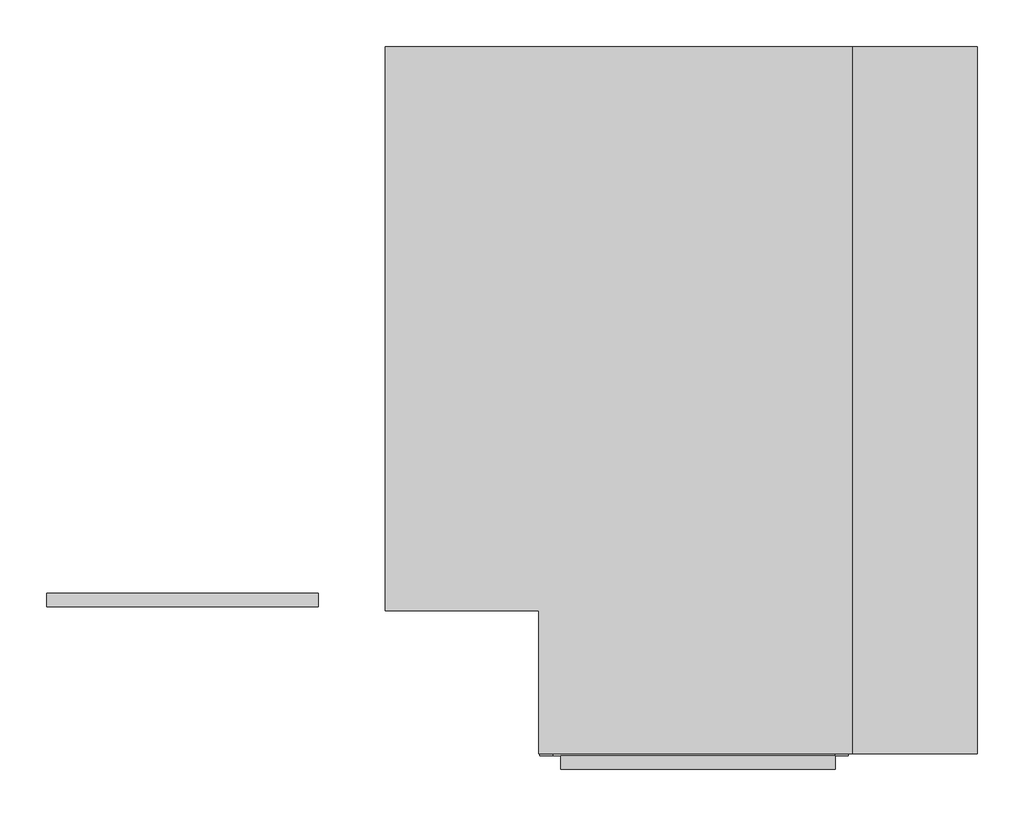
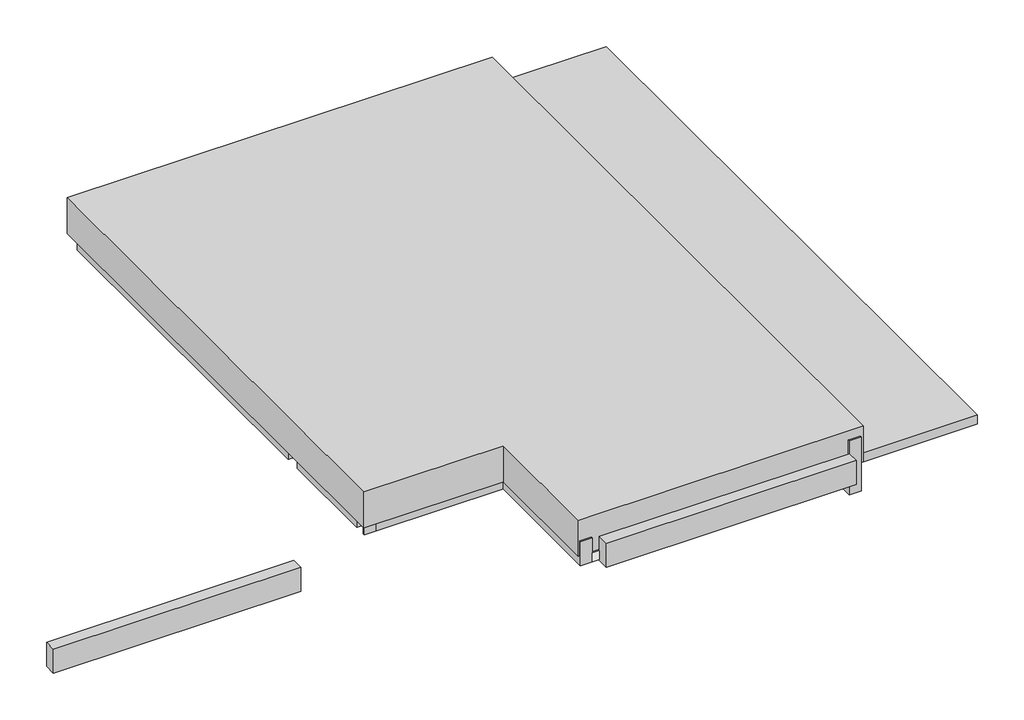
# One storey: 7 beams, 2 proxies, 2 slabs, 1 column.
"""IFC4 building model written with IfcOpenShell, lengths in millimetres."""

import ifcopenshell
import ifcopenshell.guid

model = None  # the IFC model being written
_history = None  # IfcOwnerHistory: only IFC2X3 demands one
_inside = {}  # id of a spatial element -> (the spatial element, [elements in it])
_under = {}  # id of a project, library or spatial element -> (it, [spatial elements below it])
_declared = {}  # id of a project -> (the project, [libraries it declares])
_typed = {}  # id of a type object -> (the type object, [elements of that type])
_made_of = {}  # id of a material, layer set ... -> (it, [elements and type objects made of it])


def new_model(schema):
    """Start an empty IFC model of exactly this schema.

    Asked for "IFC4X3", IfcOpenShell would pick the latest addendum, in which some entities
    have other attributes; the version numbers below select the first issue.
    IFC2X3 requires an IfcOwnerHistory on every rooted entity: one is made here for all.
    """
    global model, _history
    if schema == "IFC4X3":
        model = ifcopenshell.file(schema_version=(4, 3, 0, 0))
    else:
        model = ifcopenshell.file(schema=schema)
    _inside.clear()
    _under.clear()
    _declared.clear()
    _typed.clear()
    _made_of.clear()
    _history = None
    if model.schema == "IFC2X3":
        org = make("IfcOrganization", Name="unknown")
        user = make(
            "IfcPersonAndOrganization",
            ThePerson=make("IfcPerson", FamilyName="unknown"),
            TheOrganization=org,
        )
        app = make(
            "IfcApplication",
            ApplicationDeveloper=org,
            Version="unknown",
            ApplicationFullName="unknown",
            ApplicationIdentifier="unknown",
        )
        _history = make(
            "IfcOwnerHistory",
            OwningUser=user,
            OwningApplication=app,
            ChangeAction="ADDED",
            CreationDate=0,
        )
    return model


def make(cls, **values):
    """One entity of the class cls with the attributes given. An attribute that is None is left unset."""
    return model.create_entity(
        cls, **{name: value for name, value in values.items() if value is not None}
    )


def rooted(cls, **values):
    """An entity with a GlobalId (a new one), such as an element, a storey or a relation."""
    return make(cls, GlobalId=ifcopenshell.guid.new(), OwnerHistory=_history, **values)


def si_unit(unit_type, name, prefix=None):
    """IfcSIUnit, for example si_unit("LENGTHUNIT", "METRE", prefix="MILLI")."""
    return make("IfcSIUnit", UnitType=unit_type, Prefix=prefix, Name=name)


def assignment(units):
    """IfcUnitAssignment: the units of a project."""
    return None if units is None else make("IfcUnitAssignment", Units=units)


def point(xyz):
    """IfcCartesianPoint."""
    return None if xyz is None else make("IfcCartesianPoint", Coordinates=xyz)


def direction(xyz):
    """IfcDirection."""
    return None if xyz is None else make("IfcDirection", DirectionRatios=xyz)


def frame(location, z_axis=None, x_axis=None):
    """IfcAxis2Placement3D, a coordinate frame: its origin and axes. An axis left out is left unset."""
    return make(
        "IfcAxis2Placement3D",
        Location=point(location),
        Axis=direction(z_axis),
        RefDirection=direction(x_axis),
    )


def origin():
    """The frame at (0, 0, 0) with its axes left unset."""
    return frame((0.0, 0.0, 0.0))


def place(relative_to, where):
    """IfcLocalPlacement: puts the frame where relative to a parent placement (None: the world)."""
    return make(
        "IfcLocalPlacement", PlacementRelTo=relative_to, RelativePlacement=where
    )


def context(
    kind, dimensions, precision=None, world=None, true_north=None, identifier=None
):
    """IfcGeometricRepresentationContext, for example the 3D "Model" context."""
    return make(
        "IfcGeometricRepresentationContext",
        ContextIdentifier=identifier,
        ContextType=kind,
        CoordinateSpaceDimension=dimensions,
        Precision=precision,
        WorldCoordinateSystem=world,
        TrueNorth=true_north,
    )


def project(units=None, contexts=None):
    """IfcProject with its units and contexts."""
    return rooted(
        "IfcProject",
        Name="project",
        RepresentationContexts=contexts,
        UnitsInContext=assignment(units),
    )


def spatial(cls, under=None, at=None, **own):
    """A site, building, storey or space (cls), placed at a placement, below another one or the project."""
    s = rooted(cls, ObjectPlacement=at, **own)
    if under is not None:
        _under.setdefault(under.id(), (under, []))[1].append(s)
    return s


def polyline(points):
    """IfcPolyline through the points."""
    return make("IfcPolyline", Points=[point(p) for p in points])


def outline(outer, holes=None, kind="AREA"):
    """IfcArbitraryClosedProfileDef: a profile drawn as a closed curve; with holes, ...WithVoids."""
    if holes is None:
        return make("IfcArbitraryClosedProfileDef", ProfileType=kind, OuterCurve=outer)
    return make(
        "IfcArbitraryProfileDefWithVoids",
        ProfileType=kind,
        OuterCurve=outer,
        InnerCurves=holes,
    )


def extrude(swept, where, along, depth):
    """IfcExtrudedAreaSolid: the profile swept, set in the frame where, extruded along a direction by depth."""
    return make(
        "IfcExtrudedAreaSolid",
        SweptArea=swept,
        Position=where,
        ExtrudedDirection=direction(along),
        Depth=depth,
    )


def faces_of(points, faces, orient=None, outer=None):
    """IfcFace entities. A face is a list of loops; a loop is a list of indices into points, from 0.

    orient and outer hold one flag for each loop. By default every Orientation is true, the
    first loop of a face is its IfcFaceOuterBound and the others are IfcFaceBound.
    """
    made = []
    for i, loops in enumerate(faces):
        bounds = []
        for j, loop in enumerate(loops):
            is_outer = j == 0 if outer is None else outer[i][j]
            bounds.append(
                make(
                    "IfcFaceOuterBound" if is_outer else "IfcFaceBound",
                    Bound=make("IfcPolyLoop", Polygon=[points[k] for k in loop]),
                    Orientation=True if orient is None else orient[i][j],
                )
            )
        made.append(make("IfcFace", Bounds=bounds))
    return made


def faceted_brep(points, faces, orient=None, outer=None, voids=None):
    """IfcFacetedBrep: a solid bounded by flat faces; with voids (closed shells), ...WithVoids."""
    shared = [point(p) for p in points]
    hull = make("IfcClosedShell", CfsFaces=faces_of(shared, faces, orient, outer))
    if voids is None:
        return make("IfcFacetedBrep", Outer=hull)
    return make(
        "IfcFacetedBrepWithVoids",
        Outer=hull,
        Voids=[
            make(cls, CfsFaces=faces_of(shared, fs, o, b)) for cls, fs, o, b in voids
        ],
    )


def shape(context_of_items, identifier, shape_type, items):
    """IfcShapeRepresentation: the items that make up one representation, for example the "Body"."""
    return make(
        "IfcShapeRepresentation",
        ContextOfItems=context_of_items,
        RepresentationIdentifier=identifier,
        RepresentationType=shape_type,
        Items=items,
    )


def source(mapping_origin, context_of_items, identifier, shape_type, items):
    """IfcRepresentationMap: a shape defined once, which mapped items show again and again."""
    return make(
        "IfcRepresentationMap",
        MappingOrigin=mapping_origin,
        MappedRepresentation=shape(context_of_items, identifier, shape_type, items),
    )


def transform(
    local_origin,
    x_axis=None,
    y_axis=None,
    z_axis=None,
    scale=None,
    scale2=None,
    scale3=None,
    uniform=True,
):
    """IfcCartesianTransformationOperator3D, or its non-uniform kind. x_axis, y_axis, z_axis: its Axis1, 2, 3."""
    if uniform:
        return make(
            "IfcCartesianTransformationOperator3D",
            Axis1=direction(x_axis),
            Axis2=direction(y_axis),
            LocalOrigin=point(local_origin),
            Scale=scale,
            Axis3=direction(z_axis),
        )
    return make(
        "IfcCartesianTransformationOperator3DnonUniform",
        Axis1=direction(x_axis),
        Axis2=direction(y_axis),
        LocalOrigin=point(local_origin),
        Scale=scale,
        Axis3=direction(z_axis),
        Scale2=scale2,
        Scale3=scale3,
    )


def mapped(mapping_source, mapping_target):
    """IfcMappedItem: shows the shape of a source again, moved by a transform."""
    return make(
        "IfcMappedItem", MappingSource=mapping_source, MappingTarget=mapping_target
    )


def made_of(thing, what):
    """Note that an element or type object is made of a material, layer set ...; save() writes the relation."""
    if what is not None:
        _made_of.setdefault(what.id(), (what, []))[1].append(thing)
    return thing


def element(
    cls,
    number,
    at=None,
    inside=None,
    cuts=None,
    type_object=None,
    material=None,
    context=None,
    identifier="Body",
    shape_type=None,
    held_by="IfcProductDefinitionShape",
    body=None,
    shapes=None,
    **own,
):
    """One element of the class cls, such as IfcWall. Its Tag is "e" and its number.

    at: its placement. inside: the storey or other place that contains it. cuts: it is an
    opening in that element (IfcRelVoidsElement). A single representation is given by context,
    identifier, shape_type and body (its items); several are given by shapes. held_by: the class
    of the entity that holds the representations. save() writes the other relations.
    """
    e = rooted(cls, Tag="e%d" % number, ObjectPlacement=at, **own)
    if body is not None:
        shapes = [shape(context, identifier, shape_type, body)]
    if shapes is not None:
        e.Representation = make(held_by, Representations=shapes)
    if inside is not None:
        _inside.setdefault(inside.id(), (inside, []))[1].append(e)
    if cuts is not None:
        rooted(
            "IfcRelVoidsElement", RelatingBuildingElement=cuts, RelatedOpeningElement=e
        )
    if type_object is not None:
        _typed.setdefault(type_object.id(), (type_object, []))[1].append(e)
    return made_of(e, material)


def aggregate(whole, parts):
    """IfcRelAggregates: a whole, such as a stair, and the parts it consists of."""
    return rooted("IfcRelAggregates", RelatingObject=whole, RelatedObjects=parts)


def save(model, path):
    """Write the relations noted so far, then the file.

    IfcRelAggregates (storeys below a building ...), IfcRelContainedInSpatialStructure (elements
    in a storey), IfcRelDefinesByType, IfcRelAssociatesMaterial and IfcRelDeclares: one each for
    every whole, place, type object, material and project.
    """
    for whole, parts in _under.values():
        aggregate(whole, parts)
    for where, things in _inside.values():
        rooted(
            "IfcRelContainedInSpatialStructure",
            RelatedElements=things,
            RelatingStructure=where,
        )
    for kind, things in _typed.values():
        rooted("IfcRelDefinesByType", RelatedObjects=things, RelatingType=kind)
    for what, things in _made_of.values():
        rooted("IfcRelAssociatesMaterial", RelatedObjects=things, RelatingMaterial=what)
    for by, libraries in _declared.values():
        rooted("IfcRelDeclares", RelatingContext=by, RelatedDefinitions=libraries)
    model.write(path)


def column_f3930958(model_context):
    return source(origin(), model_context, "Body", "SweptSolid", [
        extrude(outline(polyline([(30.0, 80.0), (30.0, -80.0), (-30.0, -80.0), (-30.0, 80.0), (30.0, 80.0)])), frame((0.0, 0.0, 4460.0), z_axis=(0.0, 0.0, 1.0), x_axis=(1.0, 0.0, 0.0)), (0.0, 0.0, 1.0), 522.9),
    ])


model = new_model("IFC4")

# Units and contexts
model_context = context("Model", 3, world=origin())
ifc_project = project(units=[si_unit("LENGTHUNIT", "METRE", prefix="MILLI")], contexts=[model_context])

# Site, building, storey
site = spatial("IfcSite", under=ifc_project)
building = spatial("IfcBuilding", under=site)
storey = spatial("IfcBuildingStorey", under=building, Name="COBERTURA SALA DE ESTAR", Elevation=4400.0)

# Beams
placement = place(None, origin())
element("IfcBeam", 1, ObjectType="TQS - Viga retangular : 19.0 x 40.0", at=placement, inside=storey, context=model_context, shape_type="SweptSolid", body=[
    extrude(outline(polyline([(-7621.281307, -2044.5699847), (-7621.281307, -2234.5699847), (-11521.281307, -2234.5699847), (-11521.281307, -2044.5699847), (-7621.281307, -2044.5699847)])), frame((0.0, 0.0, 3640.0), z_axis=(0.0, 0.0, 1.0), x_axis=(1.0, 0.0, 0.0)), (0.0, 0.0, 1.0), 400.0),
])
element("IfcBeam", 2, ObjectType="TQS - Viga retangular : 19.0 x 40.0", at=placement, inside=storey, context=model_context, shape_type="SweptSolid", body=[
    extrude(outline(polyline([(-202.281307, -4375.5699847), (-202.281307, -4565.5699847), (-4142.481307, -4565.5699847), (-4142.481307, -4375.5699847), (-202.281307, -4375.5699847)])), frame((0.0, 0.0, 4240.0), z_axis=(0.0, 0.0, 1.0), x_axis=(1.0, 0.0, 0.0)), (0.0, 0.0, 1.0), 400.0),
])
element("IfcBeam", 3, ObjectType="TQS - Viga retangular : 19.0 x 40.0", at=placement, inside=storey, context=model_context, shape_type="Brep", body=[
    faceted_brep([(-4442.481307, -2259.5699847, 4650.0), (-4252.481307, -2259.5699847, 4650.0), (-4252.481307, -2259.5699847, 4400.0), (-4252.481307, -2259.5699847, 4250.0), (-4442.481307, -2259.5699847, 4250.0), (-4442.481307, -4375.5699847, 4650.0), (-4252.481307, -4375.5699847, 4650.0), (-4252.481307, -4375.5699847, 4400.0), (-4252.481307, -4375.5699847, 4250.0), (-4442.481307, -4375.5699847, 4250.0)], [[[0, 1, 2, 3, 4]], [[1, 0, 5, 6]], [[3, 2, 1, 6, 7, 8]], [[4, 3, 8, 9]], [[0, 4, 9, 5]], [[5, 9, 8, 7, 6]]]),
])
element("IfcBeam", 4, ObjectType="TQS - Viga retangular : 19.0 x 60.0", at=placement, inside=storey, context=model_context, shape_type="SweptSolid", body=[
    extrude(outline(polyline([(-412.281307, 5584.4300153), (-6230.281307, 5584.4300153), (-6230.281307, 5774.4300153), (-412.281307, 5774.4300153), (-412.281307, 5584.4300153)])), frame((0.0, 0.0, 4250.0), z_axis=(0.0, 0.0, 1.0), x_axis=(1.0, 0.0, 0.0)), (0.0, 0.0, 1.0), 600.0),
])
element("IfcBeam", 5, ObjectType="TQS - Viga retangular : 19.0 x 60.0", at=placement, inside=storey, context=model_context, shape_type="Brep", body=[
    faceted_brep([(-6630.281307, -174.5699847, 4850.0), (-6440.281307, -174.5699847, 4850.0), (-6440.281307, 5584.4300153, 4850.0), (-6630.281307, 5584.4300153, 4850.0), (-6440.281307, -174.5699847, 4250.0), (-6440.281307, 5584.4300153, 4250.0), (-6440.281307, 5584.4300153, 4400.0), (-6630.281307, -174.5699847, 4250.0), (-6630.281307, 5584.4300153, 4250.0)], [[[0, 1, 2, 3]], [[1, 4, 5, 6, 2]], [[4, 7, 8, 5]], [[7, 0, 3, 8]], [[1, 0, 7, 4]], [[3, 2, 6, 5, 8]]]),
    faceted_brep([(-6630.281307, -424.5699847, 4850.0), (-6440.281307, -424.5699847, 4850.0), (-6440.281307, -424.5699847, 4250.0), (-6630.281307, -424.5699847, 4250.0), (-6630.281307, -2044.5699847, 4850.0), (-6440.281307, -2044.5699847, 4850.0), (-6440.281307, -2044.5699847, 4250.0), (-6630.281307, -2044.5699847, 4250.0)], [[[0, 1, 2, 3]], [[1, 0, 4, 5]], [[2, 1, 5, 6]], [[3, 2, 6, 7]], [[0, 3, 7, 4]], [[5, 4, 7, 6]]]),
    faceted_brep([(-6440.281307, -2259.5699847, 4850.0), (-6630.281307, -2259.5699847, 4850.0), (-6630.281307, -2259.5699847, 4250.0), (-6440.281307, -2259.5699847, 4250.0), (-6630.281307, -2234.5699847, 4850.0), (-6440.281307, -2234.5699847, 4850.0), (-6440.281307, -2234.5699847, 4250.0), (-6630.281307, -2234.5699847, 4250.0)], [[[0, 1, 2, 3]], [[4, 5, 6, 7]], [[1, 0, 5, 4]], [[0, 3, 6, 5]], [[3, 2, 7, 6]], [[2, 1, 4, 7]]]),
])
element("IfcBeam", 6, ObjectType="TQS - Viga retangular : 19.0 x 60.0", at=placement, inside=storey, context=model_context, shape_type="Brep", body=[
    faceted_brep([(-202.6220088, -2259.5699847, 4850.0), (-202.6137562, -2069.5699847, 4850.0), (-6440.281307, -2069.5699847, 4850.0), (-6440.281307, -2234.5699847, 4850.0), (-6440.281307, -2259.5699847, 4850.0), (-202.6220088, -2259.5699847, 4250.0), (-202.6220088, -2259.5699847, 4400.0), (-6440.281307, -2259.5699847, 4250.0), (-4442.481307, -2259.5699847, 4250.0), (-4252.481307, -2259.5699847, 4250.0), (-202.6137562, -2069.5699847, 4250.0), (-6440.281307, -2234.5699847, 4250.0), (-6440.281307, -2069.5699847, 4250.0), (-202.6137562, -2069.5699847, 4400.0), (-6440.281307, -2069.5699847, 4400.0)], [[[0, 1, 2, 3, 4]], [[5, 6, 0, 4, 7, 8, 9]], [[10, 5, 9, 8, 7, 11, 12]], [[1, 13, 10, 12, 14, 2]], [[2, 14, 12, 11, 7, 4, 3]], [[1, 0, 6, 5, 10, 13]]]),
])
element("IfcBeam", 7, ObjectType="TQS - Viga retangular : 19.0 x 90.0", at=placement, inside=storey, context=model_context, shape_type="Brep", body=[
    faceted_brep([(-12.281307, 5584.4300153, 4850.0), (-202.2813068, 5584.4382679, 4850.0), (-202.6137562, -2069.5699847, 4850.0), (-202.6220088, -2259.5699847, 4850.0), (-202.7139163, -4375.561732, 4850.0), (-12.7139164, -4375.5699846, 4850.0), (-12.281307, 5584.4300153, 3950.0), (-12.7139164, -4375.5699846, 3950.0), (-202.2813068, 5584.4382679, 3950.0), (-202.7139163, -4375.561732, 3950.0)], [[[0, 1, 2, 3, 4, 5]], [[6, 0, 5, 7]], [[8, 6, 7, 9]], [[1, 8, 9, 4, 3, 2]], [[1, 0, 6, 8]], [[4, 9, 7, 5]]]),
])

# Proxies
element("IfcBuildingElementProxy", 8, Name="PERGOLADO SALAS1 : PERGOLADO SALAS", ObjectType="PERGOLADO SALAS1 : PERGOLADO SALAS", at=placement, inside=storey, context=model_context, shape_type="SweptSolid", body=[
    extrude(outline(polyline([(1839.718693, 5804.4300153), (1839.718693, -4345.5699847), (39.718693, -4345.5699847), (39.718693, 5804.4300153), (1839.718693, 5804.4300153)])), frame((0.0, 0.0, 4400.0), z_axis=(0.0, 0.0, 1.0), x_axis=(1.0, 0.0, 0.0)), (0.0, 0.0, 1.0), 150.0),
])
element("IfcBuildingElementProxy", 9, Name="COBERTURA SALA DE ESTAR : COBERTURA SALA DE ESTAR", ObjectType="COBERTURA SALA DE ESTAR : COBERTURA SALA DE ESTAR", at=placement, inside=storey, context=model_context, shape_type="SweptSolid", body=[
    extrude(outline(polyline([(39.718693, 5804.4300153), (39.718693, -4345.5699847), (-4457.4976512, -4345.5699847), (-4457.4976512, -2295.5699847), (-6660.281307, -2295.5699847), (-6660.281307, 5804.4300153), (39.718693, 5804.4300153)])), frame((0.0, 0.0, 4400.0), z_axis=(0.0, 0.0, 1.0), x_axis=(1.0, 0.0, 0.0)), (0.0, 0.0, 1.0), 600.0),
])

# Column
column_shape = column_f3930958(model_context)
element("IfcColumn", 10, ObjectType="Madeira de lei-Coluna : Pontalete 6X16cm", at=placement, inside=storey, context=model_context, shape_type="MappedRepresentation", body=[
    mapped(column_shape, transform((-3340.781307, 623.9300153, 0.0), x_axis=(1.0, 0.0, 0.0), y_axis=(0.0, 1.0, 0.0), z_axis=(0.0, 0.0, 1.0))),
])

# Slabs
element("IfcSlab", 11, ObjectType="TQS h=15", at=placement, inside=storey, context=model_context, shape_type="Brep", body=[
    faceted_brep([(-6440.281307, -2069.5699847, 4250.0), (-6440.281307, -2044.5699847, 4250.0), (-6440.281307, -424.5699847, 4250.0), (-6440.281307, -174.5699847, 4250.0), (-6440.281307, 5584.4300153, 4250.0), (-6230.281307, 5584.4300153, 4250.0), (-412.281307, 5584.4300153, 4250.0), (-202.2813071, 5584.4300153, 4250.0), (-202.6137562, -2069.5699847, 4250.0), (-6440.281307, -2069.5699847, 4400.0), (-202.6137562, -2069.5699847, 4400.0), (-202.2813071, 5584.4300153, 4400.0), (-6440.281307, 5584.4300153, 4400.0)], [[[0, 1, 2, 3, 4, 5, 6, 7, 8]], [[9, 10, 11, 12]], [[4, 3, 2, 1, 0, 9, 12]], [[7, 6, 5, 4, 12, 11]], [[8, 7, 11, 10]], [[0, 8, 10, 9]]]),
])
element("IfcSlab", 12, ObjectType="TQS h=15", at=placement, inside=storey, context=model_context, shape_type="SweptSolid", body=[
    extrude(outline(polyline([(-202.6220088, -2259.5699847), (-202.7139166, -4375.5699847), (-4252.481307, -4375.5699847), (-4252.481307, -2259.5699847), (-202.6220088, -2259.5699847)])), frame((0.0, 0.0, 4250.0), z_axis=(0.0, 0.0, 1.0), x_axis=(1.0, 0.0, 0.0)), (0.0, 0.0, 1.0), 150.0),
])

save(model, "model.ifc")

# Revit data of these elements
# Type "TQS - Viga retangular : 19.0 x 40.0"
#   Length [instance default] = 1.524 m
#   b = 0.19 m
#   h = 0.40 m
#   Structural Material [instance default] = none
#   Assembly Code = ""
# Type "TQS - Viga retangular : 19.0 x 60.0"
#   Length [instance default] = 1.524 m
#   b = 0.19 m
#   h = 0.60 m
#   Structural Material [instance default] = none
#   Assembly Code = ""
# Type "TQS - Viga retangular : 19.0 x 90.0"
#   Length [instance default] = 1.524 m
#   b = 0.19 m
#   h = 0.90 m
#   Structural Material [instance default] = none
#   Assembly Code = ""
# Type "Madeira de lei-Coluna : Pontalete 6X16cm"
#   A = 0.01952 m²
#   b = 0.06 m
#   d = 0.16 m
#   Structural Material [instance default] = none
#   Assembly Code = ""
# Type "TQS h=15"
#   Function = 0
#   Layers, outside or top first: 0.15 m ".MATERIAL GENÉRICO LAJE E PISO" (function 1)
# Element 1 (IfcBeam, "TQS - Viga retangular : 19.0 x 40.0")
#   Uso = "ESTRUTURA"
#   Titulo = "V302"
#   Chave = "-194"
#   Tipo Elemento = "Viga"
#   SHA1 = "623FD7AF7D5DA8F9D9CA08F45AA7E3989112ED0B"
#   Revisão = ""
#   Tipo de carga = ""
#   Divisor de flexao = ""
#   Secao = ""
#   Configuracao = ""
#   Angulo (graus) = ""
#   Detalhamento = ""
#   Casos de vento manual = ""
#   Tipo = ""
#   Alcas = ""
#   Furos = ""
#   Pino = ""
#   Distribuicao = ""
#   Solidarizado = ""
#   Solidarizar na montagem = ""
#   Unir com o próximo = ""
#   Grupo pre moldado = ""
#   Verificado = ""
#   Concreto C = ""
#   Taxa de armadura (kgf/m³) = 0
#   Carga (tf/m²) = 0
#   Carga (tf/m) = 0
#   Carga (tf) = 0
#   Altura = 0.40 m
#   Rebaixo = 0.36 m
#   Largura = 0.19 m
#   Distancia a face = 0.00 m
#   Distancia ao eixo = 0.00 m
#   Altura gerber esquerda = 0.00 m
#   Largura gerber esquerda = 0.00 m
#   Altura gerber direita = 0.00 m
#   Largura gerber direita = 0.00 m
#   Resultado de Ensaios fck (MPa) = 0
#   Unique TQS ID = -194
#   Principal = yes
#   Structural Material = none
#   Phase Created = CC_AP/ESTR
# Element 2 (IfcBeam, "TQS - Viga retangular : 19.0 x 40.0")
#   Uso = "ESTRUTURA"
#   Titulo = "V304"
#   Chave = "-347"
#   Tipo Elemento = "Viga"
#   SHA1 = "DE726C8B00042777CE20FAEC480409A8753BC175"
#   Revisão = ""
#   Tipo de carga = ""
#   Divisor de flexao = ""
#   Secao = ""
#   Configuracao = ""
#   Angulo (graus) = ""
#   Detalhamento = ""
#   Casos de vento manual = ""
#   Tipo = ""
#   Alcas = ""
#   Furos = ""
#   Pino = ""
#   Distribuicao = ""
#   Solidarizado = ""
#   Solidarizar na montagem = ""
#   Unir com o próximo = ""
#   Grupo pre moldado = ""
#   Verificado = ""
#   Concreto C = ""
#   Taxa de armadura (kgf/m³) = 0
#   Carga (tf/m²) = 0
#   Carga (tf/m) = 0
#   Carga (tf) = 0
#   Altura = 0.40 m
#   Rebaixo = -0.24 m
#   Largura = 0.19 m
#   Distancia a face = 0.00 m
#   Distancia ao eixo = 0.00 m
#   Altura gerber esquerda = 0.00 m
#   Largura gerber esquerda = 0.00 m
#   Altura gerber direita = 0.00 m
#   Largura gerber direita = 0.00 m
#   Resultado de Ensaios fck (MPa) = 0
#   Unique TQS ID = -347
#   Principal = yes
#   Structural Material = none
#   Phase Created = CC_AP/ESTR
# Element 3 (IfcBeam, "TQS - Viga retangular : 19.0 x 40.0")
#   Uso = "ESTRUTURA"
#   Titulo = "V306"
#   Chave = "-348"
#   Tipo Elemento = "Viga"
#   SHA1 = "0486A55721C7CA422F82DF13CBABE904850BDE6D"
#   Revisão = ""
#   Tipo de carga = ""
#   Divisor de flexao = ""
#   Secao = ""
#   Configuracao = ""
#   Angulo (graus) = ""
#   Detalhamento = ""
#   Casos de vento manual = ""
#   Tipo = ""
#   Alcas = ""
#   Furos = ""
#   Pino = ""
#   Distribuicao = ""
#   Solidarizado = ""
#   Solidarizar na montagem = ""
#   Unir com o próximo = ""
#   Grupo pre moldado = ""
#   Verificado = ""
#   Concreto C = ""
#   Taxa de armadura (kgf/m³) = 0
#   Carga (tf/m²) = 0
#   Carga (tf/m) = 0
#   Carga (tf) = 0
#   Altura = 0.40 m
#   Rebaixo = -0.25 m
#   Largura = 0.19 m
#   Distancia a face = 0.00 m
#   Distancia ao eixo = 0.00 m
#   Altura gerber esquerda = 0.00 m
#   Largura gerber esquerda = 0.00 m
#   Altura gerber direita = 0.00 m
#   Largura gerber direita = 0.00 m
#   Resultado de Ensaios fck (MPa) = 0
#   Unique TQS ID = -348
#   Principal = yes
#   Structural Material = none
#   Phase Created = CC_AP/ESTR
# Element 4 (IfcBeam, "TQS - Viga retangular : 19.0 x 60.0")
#   Uso = "ESTRUTURA"
#   Titulo = "V301"
#   Chave = "-296"
#   Tipo Elemento = "Viga"
#   SHA1 = "757894CEA72A4CB6221DF2E576041B09F085C368"
#   Revisão = ""
#   Tipo de carga = ""
#   Divisor de flexao = ""
#   Secao = ""
#   Configuracao = ""
#   Angulo (graus) = ""
#   Detalhamento = ""
#   Casos de vento manual = ""
#   Tipo = ""
#   Alcas = ""
#   Furos = ""
#   Pino = ""
#   Distribuicao = ""
#   Solidarizado = ""
#   Solidarizar na montagem = ""
#   Unir com o próximo = ""
#   Grupo pre moldado = ""
#   Verificado = ""
#   Concreto C = ""
#   Taxa de armadura (kgf/m³) = 0
#   Carga (tf/m²) = 0
#   Carga (tf/m) = 0
#   Carga (tf) = 0
#   Altura = 0.60 m
#   Rebaixo = -0.45 m
#   Largura = 0.19 m
#   Distancia a face = 0.00 m
#   Distancia ao eixo = 0.00 m
#   Altura gerber esquerda = 0.00 m
#   Largura gerber esquerda = 0.00 m
#   Altura gerber direita = 0.00 m
#   Largura gerber direita = 0.00 m
#   Resultado de Ensaios fck (MPa) = 0
#   Unique TQS ID = -296
#   Principal = yes
#   Structural Material = none
#   Phase Created = CC_AP/ESTR
# Element 5 (IfcBeam, "TQS - Viga retangular : 19.0 x 60.0")
#   Uso = "ESTRUTURA"
#   Titulo = "V305"
#   Chave = "-297"
#   Tipo Elemento = "Viga"
#   SHA1 = "BDE1024E341324ECB798242B9C26029271E807E6"
#   Revisão = ""
#   Tipo de carga = ""
#   Divisor de flexao = ""
#   Secao = ""
#   Configuracao = ""
#   Angulo (graus) = ""
#   Detalhamento = ""
#   Casos de vento manual = ""
#   Tipo = ""
#   Alcas = ""
#   Furos = ""
#   Pino = ""
#   Distribuicao = ""
#   Solidarizado = ""
#   Solidarizar na montagem = ""
#   Unir com o próximo = ""
#   Grupo pre moldado = ""
#   Verificado = ""
#   Concreto C = ""
#   Taxa de armadura (kgf/m³) = 0
#   Carga (tf/m²) = 0
#   Carga (tf/m) = 0
#   Carga (tf) = 0
#   Altura = 0.60 m
#   Rebaixo = -0.45 m
#   Largura = 0.19 m
#   Distancia a face = 0.00 m
#   Distancia ao eixo = 0.00 m
#   Altura gerber esquerda = 0.00 m
#   Largura gerber esquerda = 0.00 m
#   Altura gerber direita = 0.00 m
#   Largura gerber direita = 0.00 m
#   Resultado de Ensaios fck (MPa) = 0
#   Unique TQS ID = -297
#   Principal = yes
#   Structural Material = none
#   Phase Created = CC_AP/ESTR
# Element 6 (IfcBeam, "TQS - Viga retangular : 19.0 x 60.0")
#   Uso = "ESTRUTURA"
#   Titulo = "V303"
#   Chave = "-345"
#   Tipo Elemento = "Viga"
#   SHA1 = "033B8EC3397B601DC3ABF9BA590BF3ACBC45E410"
#   Revisão = ""
#   Tipo de carga = ""
#   Divisor de flexao = ""
#   Secao = ""
#   Configuracao = ""
#   Angulo (graus) = ""
#   Detalhamento = ""
#   Casos de vento manual = ""
#   Tipo = ""
#   Alcas = ""
#   Furos = ""
#   Pino = ""
#   Distribuicao = ""
#   Solidarizado = ""
#   Solidarizar na montagem = ""
#   Unir com o próximo = ""
#   Grupo pre moldado = ""
#   Verificado = ""
#   Concreto C = ""
#   Taxa de armadura (kgf/m³) = 0
#   Carga (tf/m²) = 0
#   Carga (tf/m) = 0
#   Carga (tf) = 0
#   Altura = 0.60 m
#   Rebaixo = -0.45 m
#   Largura = 0.19 m
#   Distancia a face = 0.00 m
#   Distancia ao eixo = 0.00 m
#   Altura gerber esquerda = 0.00 m
#   Largura gerber esquerda = 0.00 m
#   Altura gerber direita = 0.00 m
#   Largura gerber direita = 0.00 m
#   Resultado de Ensaios fck (MPa) = 0
#   Unique TQS ID = -345
#   Principal = yes
#   Structural Material = none
#   Phase Created = CC_AP/ESTR
# Element 7 (IfcBeam, "TQS - Viga retangular : 19.0 x 90.0")
#   Uso = "ESTRUTURA"
#   Titulo = "V307"
#   Chave = "-298"
#   Tipo Elemento = "Viga"
#   SHA1 = "4A4DC69E98A9D766DC72AD6B038202D9AEA1F49E"
#   Revisão = ""
#   Tipo de carga = ""
#   Divisor de flexao = ""
#   Secao = ""
#   Configuracao = ""
#   Angulo (graus) = ""
#   Detalhamento = ""
#   Casos de vento manual = ""
#   Tipo = ""
#   Alcas = ""
#   Furos = ""
#   Pino = ""
#   Distribuicao = ""
#   Solidarizado = ""
#   Solidarizar na montagem = ""
#   Unir com o próximo = ""
#   Grupo pre moldado = ""
#   Verificado = ""
#   Concreto C = ""
#   Taxa de armadura (kgf/m³) = 0
#   Carga (tf/m²) = 0
#   Carga (tf/m) = 0
#   Carga (tf) = 0
#   Altura = 0.90 m
#   Rebaixo = -0.45 m
#   Largura = 0.19 m
#   Distancia a face = 0.00 m
#   Distancia ao eixo = 0.00 m
#   Altura gerber esquerda = 0.00 m
#   Largura gerber esquerda = 0.00 m
#   Altura gerber direita = 0.00 m
#   Largura gerber direita = 0.00 m
#   Resultado de Ensaios fck (MPa) = 0
#   Unique TQS ID = -298
#   Principal = yes
#   Structural Material = none
#   Phase Created = CC_AP/ESTR
# Element 8 (IfcBuildingElementProxy, "PERGOLADO SALAS1 : PERGOLADO SALAS")
#   Phase Created = CC_COMPLETO
#   Materials on its faces: "Forma padrão"
# Element 9 (IfcBuildingElementProxy, "COBERTURA SALA DE ESTAR : COBERTURA SALA DE ESTAR")
#   Phase Created = CC_EV
#   Materials on its faces: "Forma padrão"
# Element 10 (IfcColumn, "Madeira de lei-Coluna : Pontalete 6X16cm")
#   Comments = ""
#   Structural Material = .MADEIRAMENTO
#   Phase Created = CC_PE
#   Materials on its faces: ".MADEIRAMENTO"
# Element 11 (IfcSlab, "TQS h=15")
#   Uso = "ESTRUTURA"
#   Titulo = "L1"
#   Chave = "-343"
#   Tipo Elemento = "Laje"
#   SHA1 = "CBCB75B0B1E6306AA97FD72F3CCB2019DA0CDC21"
#   Revisão = ""
#   Tipo de carga = ""
#   Divisor de flexao = ""
#   Fabricante = ""
#   Enchimento = ""
#   Mini painel = ""
#   Blocos por nervura = ""
#   Secao = ""
#   Configuracao = ""
#   Angulo (graus) = "0"
#   Detalhamento = ""
#   Casos de vento manual = ""
#   Tipo = "Pré-moldada"
#   Alcas = ""
#   Furos = ""
#   Pino = ""
#   Distribuicao = ""
#   Solidarizado = ""
#   Solidarizar na montagem = ""
#   Unir com o próximo = ""
#   Grupo pre moldado = ""
#   Verificado = ""
#   Concreto C = ""
#   Height Offset From Level = 0.00 m
#   Taxa de armadura (kgf/m³) = 0
#   Carga (tf/m²) = 0
#   Carga (tf/m) = 0
#   Carga (tf) = 0
#   Altura = 0.15 m
#   Capa = 0.04 m
#   Capa inferior = 0.00 m
#   Altura da nervura = 0.11 m
#   Enchimento (tf/m³) = 0.02
#   Largura inferior X = 0.00 m
#   Distancia inferior X = 0.00 m
#   Largura inferior Y = 0.00 m
#   Distancia inferior Y = 0.00 m
#   Largura vigota = 0.00 m
#   Altura vigota = 0.00 m
#   Largura perfil = 0.00 m
#   Largura aba = 0.00 m
#   Altura perfil = 0.00 m
#   Nervura secundaria = 0.00 m
#   Desconto nervura secundaria = 0.00 m
#   Rebaixo = 0.00 m
#   Largura = 0.00 m
#   Distancia a face = 0.00 m
#   Distancia ao eixo = 0.00 m
#   Resultado de Ensaios fck (MPa) = 0
#   built-in parameter 1001954 = 1
#   Unique TQS ID = -343
#   Principal = yes
#   Phase Created = CC_AP/ESTR
#   Materials on its faces: ".MATERIAL GENÉRICO LAJE E PISO"
# Element 12 (IfcSlab, "TQS h=15")
#   Uso = "ESTRUTURA"
#   Titulo = "L2"
#   Chave = "-344"
#   Tipo Elemento = "Laje"
#   SHA1 = "B69E32F9CB7C87F86F0BE6D4DE0B78773B0CC6FF"
#   Revisão = ""
#   Tipo de carga = ""
#   Divisor de flexao = ""
#   Fabricante = ""
#   Enchimento = ""
#   Mini painel = ""
#   Blocos por nervura = ""
#   Secao = ""
#   Configuracao = ""
#   Angulo (graus) = "90"
#   Detalhamento = ""
#   Casos de vento manual = ""
#   Tipo = "Pré-moldada"
#   Alcas = ""
#   Furos = ""
#   Pino = ""
#   Distribuicao = ""
#   Solidarizado = ""
#   Solidarizar na montagem = ""
#   Unir com o próximo = ""
#   Grupo pre moldado = ""
#   Verificado = ""
#   Concreto C = ""
#   Height Offset From Level = 0.00 m
#   Taxa de armadura (kgf/m³) = 0
#   Carga (tf/m²) = 0
#   Carga (tf/m) = 0
#   Carga (tf) = 0
#   Altura = 0.15 m
#   Capa = 0.04 m
#   Capa inferior = 0.00 m
#   Altura da nervura = 0.11 m
#   Enchimento (tf/m³) = 0.02
#   Largura inferior X = 0.00 m
#   Distancia inferior X = 0.00 m
#   Largura inferior Y = 0.00 m
#   Distancia inferior Y = 0.00 m
#   Largura vigota = 0.00 m
#   Altura vigota = 0.00 m
#   Largura perfil = 0.00 m
#   Largura aba = 0.00 m
#   Altura perfil = 0.00 m
#   Nervura secundaria = 0.00 m
#   Desconto nervura secundaria = 0.00 m
#   Rebaixo = 0.00 m
#   Largura = 0.00 m
#   Distancia a face = 0.00 m
#   Distancia ao eixo = 0.00 m
#   Resultado de Ensaios fck (MPa) = 0
#   built-in parameter 1001954 = 1
#   Unique TQS ID = -344
#   Principal = yes
#   Phase Created = CC_AP/ESTR
#   Materials on its faces: ".MATERIAL GENÉRICO LAJE E PISO"
# Materials
#   ".MATERIAL GENÉRICO LAJE E PISO": class ".CC_PAVIMENTAÇÃO", colour RGB 128 128 128, transparency 0, Description = "Material genérico para representação ND 200.", Cost = 0
#   "Forma padrão": class "Genérico", colour RGB 185 189 196, transparency 0.5, Cost = 0
#   ".MADEIRAMENTO": class ".CC_MADEIRAS", colour RGB 212 179 113, transparency 0, Cost = 0
